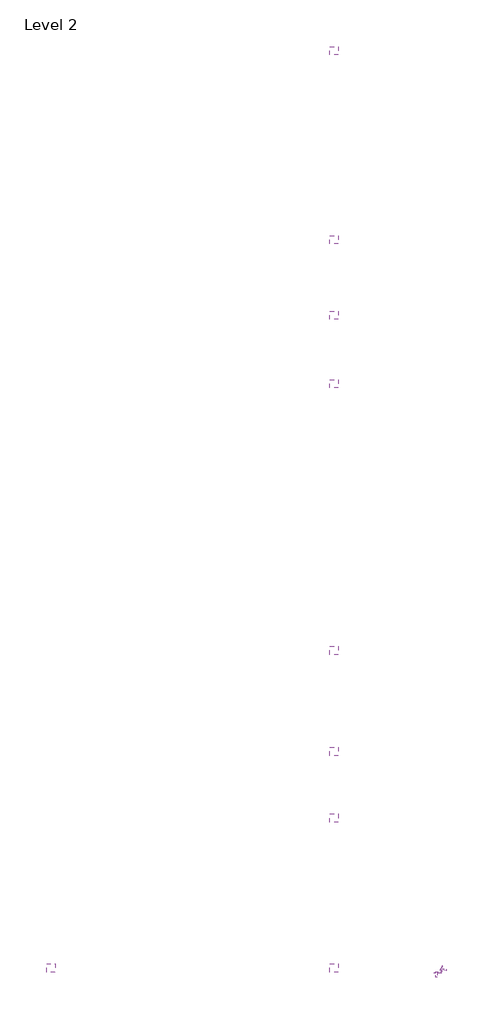
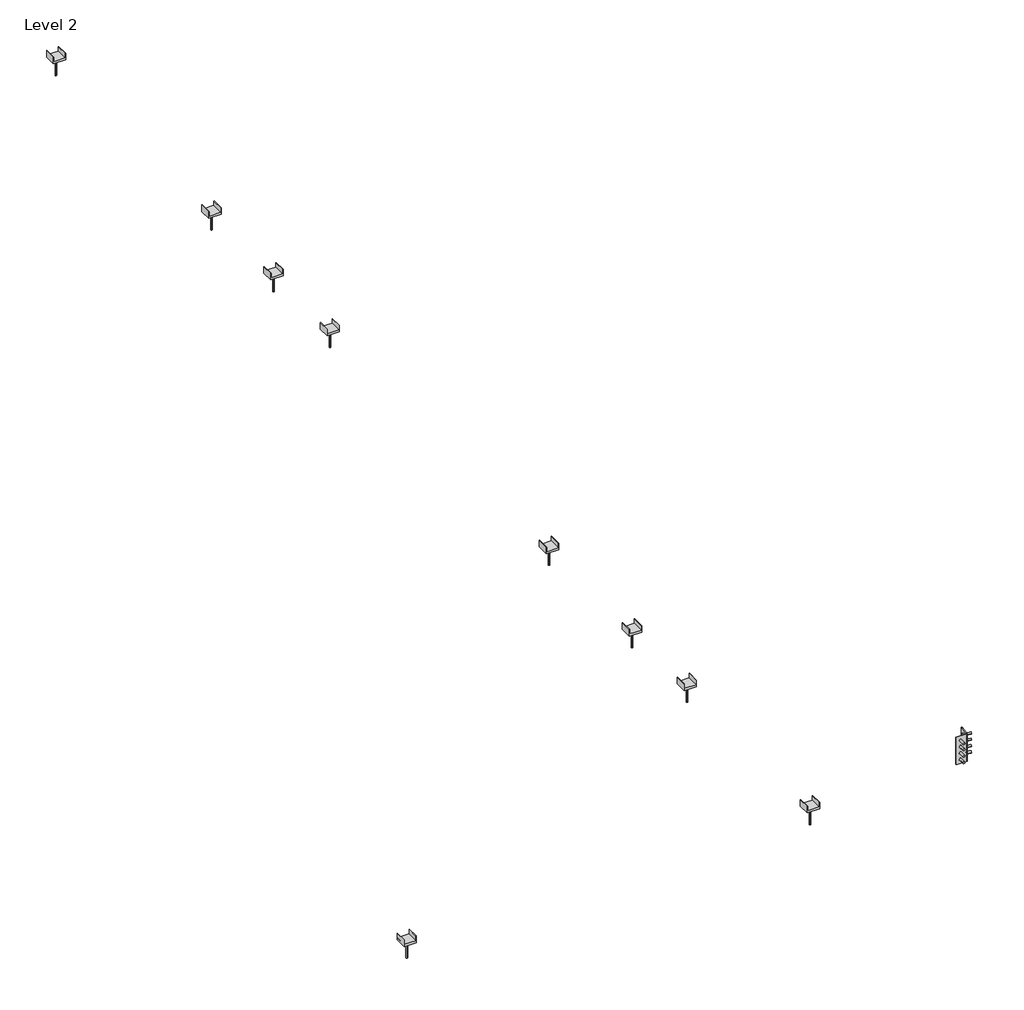
# One storey: 10 fasteners.
"""IFC4 building model written with IfcOpenShell, lengths in millimetres."""

import ifcopenshell
import ifcopenshell.guid

model = None  # the IFC model being written
_history = None  # IfcOwnerHistory: only IFC2X3 demands one
_inside = {}  # id of a spatial element -> (the spatial element, [elements in it])
_under = {}  # id of a project, library or spatial element -> (it, [spatial elements below it])
_declared = {}  # id of a project -> (the project, [libraries it declares])
_typed = {}  # id of a type object -> (the type object, [elements of that type])
_made_of = {}  # id of a material, layer set ... -> (it, [elements and type objects made of it])


def new_model(schema):
    """Start an empty IFC model of exactly this schema.

    Asked for "IFC4X3", IfcOpenShell would pick the latest addendum, in which some entities
    have other attributes; the version numbers below select the first issue.
    IFC2X3 requires an IfcOwnerHistory on every rooted entity: one is made here for all.
    """
    global model, _history
    if schema == "IFC4X3":
        model = ifcopenshell.file(schema_version=(4, 3, 0, 0))
    else:
        model = ifcopenshell.file(schema=schema)
    _inside.clear()
    _under.clear()
    _declared.clear()
    _typed.clear()
    _made_of.clear()
    _history = None
    if model.schema == "IFC2X3":
        org = make("IfcOrganization", Name="unknown")
        user = make(
            "IfcPersonAndOrganization",
            ThePerson=make("IfcPerson", FamilyName="unknown"),
            TheOrganization=org,
        )
        app = make(
            "IfcApplication",
            ApplicationDeveloper=org,
            Version="unknown",
            ApplicationFullName="unknown",
            ApplicationIdentifier="unknown",
        )
        _history = make(
            "IfcOwnerHistory",
            OwningUser=user,
            OwningApplication=app,
            ChangeAction="ADDED",
            CreationDate=0,
        )
    return model


def make(cls, **values):
    """One entity of the class cls with the attributes given. An attribute that is None is left unset."""
    return model.create_entity(
        cls, **{name: value for name, value in values.items() if value is not None}
    )


def rooted(cls, **values):
    """An entity with a GlobalId (a new one), such as an element, a storey or a relation."""
    return make(cls, GlobalId=ifcopenshell.guid.new(), OwnerHistory=_history, **values)


def si_unit(unit_type, name, prefix=None):
    """IfcSIUnit, for example si_unit("LENGTHUNIT", "METRE", prefix="MILLI")."""
    return make("IfcSIUnit", UnitType=unit_type, Prefix=prefix, Name=name)


def assignment(units):
    """IfcUnitAssignment: the units of a project."""
    return None if units is None else make("IfcUnitAssignment", Units=units)


def point(xyz):
    """IfcCartesianPoint."""
    return None if xyz is None else make("IfcCartesianPoint", Coordinates=xyz)


def direction(xyz):
    """IfcDirection."""
    return None if xyz is None else make("IfcDirection", DirectionRatios=xyz)


def frame(location, z_axis=None, x_axis=None):
    """IfcAxis2Placement3D, a coordinate frame: its origin and axes. An axis left out is left unset."""
    return make(
        "IfcAxis2Placement3D",
        Location=point(location),
        Axis=direction(z_axis),
        RefDirection=direction(x_axis),
    )


def frame_2d(location, x_axis=None):
    """IfcAxis2Placement2D, a coordinate frame in the plane: its origin and x axis."""
    return make(
        "IfcAxis2Placement2D", Location=point(location), RefDirection=direction(x_axis)
    )


def origin():
    """The frame at (0, 0, 0) with its axes left unset."""
    return frame((0.0, 0.0, 0.0))


def origin_with_axes():
    """The frame at (0, 0, 0) with the z axis (0, 0, 1) and the x axis (1, 0, 0) written out."""
    return frame((0.0, 0.0, 0.0), z_axis=(0.0, 0.0, 1.0), x_axis=(1.0, 0.0, 0.0))


def origin_2d():
    """The frame at (0, 0) in the plane with its x axis left unset."""
    return frame_2d((0.0, 0.0))


def place(relative_to, where):
    """IfcLocalPlacement: puts the frame where relative to a parent placement (None: the world)."""
    return make(
        "IfcLocalPlacement", PlacementRelTo=relative_to, RelativePlacement=where
    )


def context(
    kind, dimensions, precision=None, world=None, true_north=None, identifier=None
):
    """IfcGeometricRepresentationContext, for example the 3D "Model" context."""
    return make(
        "IfcGeometricRepresentationContext",
        ContextIdentifier=identifier,
        ContextType=kind,
        CoordinateSpaceDimension=dimensions,
        Precision=precision,
        WorldCoordinateSystem=world,
        TrueNorth=true_north,
    )


def project(units=None, contexts=None):
    """IfcProject with its units and contexts."""
    return rooted(
        "IfcProject",
        Name="project",
        RepresentationContexts=contexts,
        UnitsInContext=assignment(units),
    )


def spatial(cls, under=None, at=None, **own):
    """A site, building, storey or space (cls), placed at a placement, below another one or the project."""
    s = rooted(cls, ObjectPlacement=at, **own)
    if under is not None:
        _under.setdefault(under.id(), (under, []))[1].append(s)
    return s


def polyline(points):
    """IfcPolyline through the points."""
    return make("IfcPolyline", Points=[point(p) for p in points])


def circle_curve(where, radius):
    """IfcCircle in the frame where."""
    return make("IfcCircle", Position=where, Radius=radius)


def trimmed(basis, trim1, trim2, sense, master):
    """IfcTrimmedCurve: the piece of a basis curve between two trims."""
    return make(
        "IfcTrimmedCurve",
        BasisCurve=basis,
        Trim1=trim1,
        Trim2=trim2,
        SenseAgreement=sense,
        MasterRepresentation=master,
    )


def segment(curve, same_sense, transition):
    """IfcCompositeCurveSegment."""
    return make(
        "IfcCompositeCurveSegment",
        Transition=transition,
        SameSense=same_sense,
        ParentCurve=curve,
    )


def composite_curve(segments, self_intersect=None):
    """IfcCompositeCurve: segments joined end to end."""
    return make("IfcCompositeCurve", Segments=segments, SelfIntersect=self_intersect)


def outline(outer, holes=None, kind="AREA"):
    """IfcArbitraryClosedProfileDef: a profile drawn as a closed curve; with holes, ...WithVoids."""
    if holes is None:
        return make("IfcArbitraryClosedProfileDef", ProfileType=kind, OuterCurve=outer)
    return make(
        "IfcArbitraryProfileDefWithVoids",
        ProfileType=kind,
        OuterCurve=outer,
        InnerCurves=holes,
    )


def extrude(swept, where, along, depth):
    """IfcExtrudedAreaSolid: the profile swept, set in the frame where, extruded along a direction by depth."""
    return make(
        "IfcExtrudedAreaSolid",
        SweptArea=swept,
        Position=where,
        ExtrudedDirection=direction(along),
        Depth=depth,
    )


def shape(context_of_items, identifier, shape_type, items):
    """IfcShapeRepresentation: the items that make up one representation, for example the "Body"."""
    return make(
        "IfcShapeRepresentation",
        ContextOfItems=context_of_items,
        RepresentationIdentifier=identifier,
        RepresentationType=shape_type,
        Items=items,
    )


def source(mapping_origin, context_of_items, identifier, shape_type, items):
    """IfcRepresentationMap: a shape defined once, which mapped items show again and again."""
    return make(
        "IfcRepresentationMap",
        MappingOrigin=mapping_origin,
        MappedRepresentation=shape(context_of_items, identifier, shape_type, items),
    )


def transform(
    local_origin,
    x_axis=None,
    y_axis=None,
    z_axis=None,
    scale=None,
    scale2=None,
    scale3=None,
    uniform=True,
):
    """IfcCartesianTransformationOperator3D, or its non-uniform kind. x_axis, y_axis, z_axis: its Axis1, 2, 3."""
    if uniform:
        return make(
            "IfcCartesianTransformationOperator3D",
            Axis1=direction(x_axis),
            Axis2=direction(y_axis),
            LocalOrigin=point(local_origin),
            Scale=scale,
            Axis3=direction(z_axis),
        )
    return make(
        "IfcCartesianTransformationOperator3DnonUniform",
        Axis1=direction(x_axis),
        Axis2=direction(y_axis),
        LocalOrigin=point(local_origin),
        Scale=scale,
        Axis3=direction(z_axis),
        Scale2=scale2,
        Scale3=scale3,
    )


def mapped(mapping_source, mapping_target):
    """IfcMappedItem: shows the shape of a source again, moved by a transform."""
    return make(
        "IfcMappedItem", MappingSource=mapping_source, MappingTarget=mapping_target
    )


def made_of(thing, what):
    """Note that an element or type object is made of a material, layer set ...; save() writes the relation."""
    if what is not None:
        _made_of.setdefault(what.id(), (what, []))[1].append(thing)
    return thing


def element(
    cls,
    number,
    at=None,
    inside=None,
    cuts=None,
    type_object=None,
    material=None,
    context=None,
    identifier="Body",
    shape_type=None,
    held_by="IfcProductDefinitionShape",
    body=None,
    shapes=None,
    **own,
):
    """One element of the class cls, such as IfcWall. Its Tag is "e" and its number.

    at: its placement. inside: the storey or other place that contains it. cuts: it is an
    opening in that element (IfcRelVoidsElement). A single representation is given by context,
    identifier, shape_type and body (its items); several are given by shapes. held_by: the class
    of the entity that holds the representations. save() writes the other relations.
    """
    e = rooted(cls, Tag="e%d" % number, ObjectPlacement=at, **own)
    if body is not None:
        shapes = [shape(context, identifier, shape_type, body)]
    if shapes is not None:
        e.Representation = make(held_by, Representations=shapes)
    if inside is not None:
        _inside.setdefault(inside.id(), (inside, []))[1].append(e)
    if cuts is not None:
        rooted(
            "IfcRelVoidsElement", RelatingBuildingElement=cuts, RelatedOpeningElement=e
        )
    if type_object is not None:
        _typed.setdefault(type_object.id(), (type_object, []))[1].append(e)
    return made_of(e, material)


def aggregate(whole, parts):
    """IfcRelAggregates: a whole, such as a stair, and the parts it consists of."""
    return rooted("IfcRelAggregates", RelatingObject=whole, RelatedObjects=parts)


def save(model, path):
    """Write the relations noted so far, then the file.

    IfcRelAggregates (storeys below a building ...), IfcRelContainedInSpatialStructure (elements
    in a storey), IfcRelDefinesByType, IfcRelAssociatesMaterial and IfcRelDeclares: one each for
    every whole, place, type object, material and project.
    """
    for whole, parts in _under.values():
        aggregate(whole, parts)
    for where, things in _inside.values():
        rooted(
            "IfcRelContainedInSpatialStructure",
            RelatedElements=things,
            RelatingStructure=where,
        )
    for kind, things in _typed.values():
        rooted("IfcRelDefinesByType", RelatedObjects=things, RelatingType=kind)
    for what, things in _made_of.values():
        rooted("IfcRelAssociatesMaterial", RelatedObjects=things, RelatingMaterial=what)
    for by, libraries in _declared.values():
        rooted("IfcRelDeclares", RelatingContext=by, RelatedDefinitions=libraries)
    model.write(path)


def plane_surface(at):
    """IfcPlane: the flat surface through the origin of the frame at, square to its z axis."""
    return make("IfcPlane", Position=at)


def revolved_surface(curve, axis_point, axis_direction):
    """IfcSurfaceOfRevolution: the curve turned about the line through axis_point along axis_direction."""
    return make(
        "IfcSurfaceOfRevolution",
        SweptCurve=make("IfcArbitraryOpenProfileDef", ProfileType="CURVE", Curve=curve),
        AxisPosition=make("IfcAxis1Placement", Location=point(axis_point), Axis=direction(axis_direction)),
    )


def advanced_brep(points, edges, surfaces, faces):
    """IfcAdvancedBrep: a solid bounded by faces that lie on surfaces and meet in shared edges.

    An edge is (start, end): straight between two places in points (the first is 0);
    or (start, end, curve); or (start, end, curve, False) where it runs against its curve.
    A face is (place in surfaces, loops), or (place, loops, False) where it looks against
    its surface's normal. A loop lists edges by number (the first is 1), with a minus sign
    where the edge is run from its end to its start. The first loop is the outer one.
    """
    corners = [point(p) for p in points]
    vertices = [make("IfcVertexPoint", VertexGeometry=c) for c in corners]
    made = []
    for start, end, *more in edges:
        made.append(
            make(
                "IfcEdgeCurve",
                EdgeStart=vertices[start],
                EdgeEnd=vertices[end],
                EdgeGeometry=more[0] if more else make("IfcPolyline", Points=[corners[start], corners[end]]),
                SameSense=more[1] if len(more) > 1 else True,
            )
        )
    hull = []
    for where, loops, *sense in faces:
        bounds = []
        for j, loop in enumerate(loops):
            ring = [make("IfcOrientedEdge", EdgeElement=made[abs(k) - 1], Orientation=k > 0) for k in loop]
            bounds.append(
                make(
                    "IfcFaceOuterBound" if j == 0 else "IfcFaceBound",
                    Bound=make("IfcEdgeLoop", EdgeList=ring),
                    Orientation=True,
                )
            )
        hull.append(make("IfcAdvancedFace", Bounds=bounds, FaceSurface=surfaces[where], SameSense=sense[0] if sense else True))
    return make("IfcAdvancedBrep", Outer=make("IfcClosedShell", CfsFaces=hull))


def fastener_d5b4f6b8(model_context):
    return source(origin(), model_context, "Body", "SweptSolid", [
        extrude(outline(composite_curve([segment(trimmed(circle_curve(origin_2d(), 7.9375), [point((-7.9375, 0.0))], [point((7.9375, 0.0))], False, "CARTESIAN"), True, "CONTINUOUS"), segment(trimmed(circle_curve(origin_2d(), 7.9375), [point((7.9375, 0.0))], [point((-7.9375, 0.0))], False, "CARTESIAN"), True, "CONTINUOUS")], self_intersect=False)), frame((0.0, 0.0, -203.2), z_axis=(0.0, 0.0, 1.0), x_axis=(1.0, 0.0, 0.0)), (0.0, 0.0, 1.0), 203.2),
        extrude(outline(polyline([(-11.90625, 6.8740766), (0.0, 13.7481533), (11.90625, 6.8740766), (11.90625, -6.8740766), (0.0, -13.7481533), (-11.90625, -6.8740766), (-11.90625, 6.8740766)])), origin_with_axes(), (0.0, 0.0, 1.0), 11.2117187),
        extrude(outline(polyline([(-69.85, 79.375), (-66.675, 79.375), (-66.675, 25.4), (66.675, 25.4), (66.675, 79.375), (69.85, 79.375), (69.85, 0.0), (-69.85, 0.0), (-69.85, 79.375)])), frame((-68.2625, 0.0, 0.0), z_axis=(1.0, 0.0, 0.0), x_axis=(0.0, 1.0, 0.0)), (0.0, 0.0, 1.0), 136.525),
    ])


def fastener_ec502d19(model_context):
    return source(origin(), model_context, "Body", "SweptSolid", [
        extrude(outline(composite_curve([segment(trimmed(circle_curve(origin_2d(), 7.9375), [point((-7.9375, 0.0))], [point((7.9375, 0.0))], False, "CARTESIAN"), True, "CONTINUOUS"), segment(trimmed(circle_curve(origin_2d(), 7.9375), [point((7.9375, 0.0))], [point((-7.9375, 0.0))], False, "CARTESIAN"), True, "CONTINUOUS")], self_intersect=False)), frame((0.0, 0.0, -203.2), z_axis=(0.0, 0.0, 1.0), x_axis=(1.0, 0.0, 0.0)), (0.0, 0.0, 1.0), 203.2),
        extrude(outline(polyline([(-11.90625, -6.8740766), (-11.90625, 6.8740766), (0.0, 13.7481533), (11.90625, 6.8740766), (11.90625, -6.8740766), (0.0, -13.7481533), (-11.90625, -6.8740766)])), origin_with_axes(), (0.0, 0.0, 1.0), 11.2117187),
        extrude(outline(polyline([(69.85, 79.375), (69.85, 0.0), (-69.85, 0.0), (-69.85, 79.375), (-66.675, 79.375), (-66.675, 25.4), (66.675, 25.4), (66.675, 79.375), (69.85, 79.375)])), frame((-68.2625, 0.0, 0.0), z_axis=(1.0, 0.0, 0.0), x_axis=(0.0, 1.0, 0.0)), (0.0, 0.0, 1.0), 136.525),
    ])


def corner_bracket_angled_dba65dea(model_context):
    return source(origin(), model_context, "Body", "SolidModel", [
        advanced_brep(
        [(65.484375, -7.9375, 203.2), (65.484375, 0.0, 203.2), (93.265625, 0.0, 203.2), (93.265625, -7.9375, 203.2), (93.265625, -7.9375, 279.4), (93.265625, 0.0, 279.4), (65.484375, 0.0, 279.4), (65.484375, -7.9375, 279.4), (127.0, 0.0, 0.0), (127.0, 0.0, 330.2), (127.0, -7.9375, 330.2), (127.0, -7.9375, 0.0), (65.484375, -7.9375, 127.0), (65.484375, 0.0, 127.0), (93.265625, 0.0, 127.0), (93.265625, -7.9375, 127.0), (65.484375, -7.9375, 50.8), (65.484375, 0.0, 50.8), (93.265625, 0.0, 50.8), (93.265625, -7.9375, 50.8), (7.1469571, -7.9375, 330.2), (7.1469571, -7.9375, 0.0), (0.0, 0.0, 0.0), (0.0, 0.0, 330.2), (7.8940175, -0.8296947, 330.2), (7.8940175, -0.8296947, 0.0)],
        [
            (0, 1),
            (1, 2, circle_curve(frame((79.375, 0.0, 203.2), z_axis=(0.0, 1.0, 0.0), x_axis=(-1.0000000000000002, 0.0, 0.0)), 13.890625)),
            (2, 3),
            (3, 0, circle_curve(frame((79.375, -7.9375, 203.2), z_axis=(0.0, -1.0, 0.0), x_axis=(-1.0000000000000002, 0.0, 0.0)), 13.890625)),
            (4, 5),
            (5, 6, circle_curve(frame((79.375, 0.0, 279.4), z_axis=(0.0, 1.0, 0.0), x_axis=(-1.0000000000000002, 0.0, 0.0)), 13.890625)),
            (6, 7),
            (7, 4, circle_curve(frame((79.375, -7.9375, 279.4), z_axis=(0.0, -1.0, 0.0), x_axis=(-1.0000000000000002, 0.0, 0.0)), 13.890625)),
            (8, 9),
            (9, 10),
            (10, 11),
            (11, 8),
            (6, 5, circle_curve(frame((79.375, 0.0, 279.4), z_axis=(0.0, 1.0, 0.0), x_axis=(-1.0000000000000002, 0.0, 0.0)), 13.890625)),
            (4, 7, circle_curve(frame((79.375, -7.9375, 279.4), z_axis=(0.0, -1.0, 0.0), x_axis=(-1.0000000000000002, 0.0, 0.0)), 13.890625)),
            (12, 13),
            (13, 14, circle_curve(frame((79.375, 0.0, 127.0), z_axis=(0.0, 1.0, 0.0), x_axis=(-1.0000000000000002, 0.0, 0.0)), 13.890625)),
            (14, 15),
            (15, 12, circle_curve(frame((79.375, -7.9375, 127.0), z_axis=(0.0, -1.0, 0.0), x_axis=(-1.0000000000000002, 0.0, 0.0)), 13.890625)),
            (16, 17),
            (17, 18, circle_curve(frame((79.375, 0.0, 50.8), z_axis=(0.0, 1.0, 0.0), x_axis=(-1.0000000000000002, 0.0, 0.0)), 13.890625)),
            (18, 19),
            (19, 16, circle_curve(frame((79.375, -7.9375, 50.8), z_axis=(0.0, -1.0, 0.0), x_axis=(-1.0000000000000002, 0.0, 0.0)), 13.890625)),
            (10, 20),
            (20, 21),
            (21, 11),
            (3, 0, circle_curve(frame((79.375, -7.9375, 203.2), z_axis=(0.0, 1.0, 0.0), x_axis=(-1.0000000000000002, 0.0, 0.0)), 13.890625)),
            (15, 12, circle_curve(frame((79.375, -7.9375, 127.0), z_axis=(0.0, 1.0, 0.0), x_axis=(-1.0000000000000002, 0.0, 0.0)), 13.890625)),
            (19, 16, circle_curve(frame((79.375, -7.9375, 50.8), z_axis=(0.0, 1.0, 0.0), x_axis=(-1.0000000000000002, 0.0, 0.0)), 13.890625)),
            (8, 22),
            (22, 23),
            (23, 9),
            (1, 2, circle_curve(frame((79.375, 0.0, 203.2), z_axis=(0.0, -1.0, 0.0), x_axis=(-1.0000000000000002, 0.0, 0.0)), 13.890625)),
            (13, 14, circle_curve(frame((79.375, 0.0, 127.0), z_axis=(0.0, -1.0, 0.0), x_axis=(-1.0000000000000002, 0.0, 0.0)), 13.890625)),
            (17, 18, circle_curve(frame((79.375, 0.0, 50.8), z_axis=(0.0, -1.0, 0.0), x_axis=(-1.0000000000000002, 0.0, 0.0)), 13.890625)),
            (23, 24),
            (24, 20),
            (21, 25),
            (25, 22),
            (24, 25),
        ],
        [
            revolved_surface(polyline([(65.484375, -7.937500000000007, 203.2), (65.484375, 0.0, 203.2)]), (79.375, 0.0, 203.2), (0.0, -1.0000000000000004, 0.0)),
            revolved_surface(polyline([(65.484375, -7.937500000000007, 279.4), (65.484375, 0.0, 279.4)]), (79.375, 0.0, 279.4), (0.0, -1.0000000000000004, 0.0)),
            plane_surface(frame((127.0, -7.9375, 330.2), z_axis=(1.0, 0.0, 0.0), x_axis=(0.0, 1.0, 0.0))),
            revolved_surface(polyline([(65.484375, -7.937500000000007, 127.0), (65.484375, 0.0, 127.0)]), (79.375, 0.0, 127.0), (0.0, -1.0000000000000004, 0.0)),
            revolved_surface(polyline([(65.484375, -7.937500000000007, 50.8), (65.484375, 0.0, 50.8)]), (79.375, 0.0, 50.8), (0.0, -1.0000000000000004, 0.0)),
            plane_surface(frame((127.0, -7.9375, 330.2), z_axis=(0.0, -1.0, 0.0), x_axis=(1.0, 0.0, 0.0))),
            plane_surface(frame((127.0, 0.0, 330.2), z_axis=(0.0, 1.0, 0.0), x_axis=(-1.0, 0.0, 0.0))),
            plane_surface(frame((0.0, -7.9375, 330.2), z_axis=(0.0, 0.0, 1.0), x_axis=(0.0, 1.0, 0.0))),
            plane_surface(frame((127.0, -7.9375, 0.0), z_axis=(0.0, 0.0, -1.0), x_axis=(0.0, 1.0, 0.0))),
            plane_surface(frame((-5.3810973, -127.1339754, 330.2), z_axis=(-0.9945218953682736, 0.10452846326765133, 0.0), x_axis=(-0.10452846326765133, -0.9945218953682736, 0.0))),
            plane_surface(frame((7.8940175, -0.8296947, 0.0), z_axis=(-0.10452846326765133, -0.9945218953682736, 0.0), x_axis=(-0.9945218953682736, 0.10452846326765133, 0.0))),
        ],
        [
            (0, [[1, 2, 3, 4]]),
            (1, [[5, 6, 7, 8]]),
            (2, [[9, 10, 11, 12]]),
            (1, [[-7, 13, -5, 14]]),
            (3, [[15, 16, 17, 18]]),
            (4, [[19, 20, 21, 22]]),
            (5, [[23, 24, 25, -11], [-14, -8], [-4, 26], [-18, 27], [-22, 28]]),
            (6, [[-9, 29, 30, 31], [-2, 32], [-16, 33], [-13, -6], [-20, 34]]),
            (7, [[35, 36, -23, -10, -31]]),
            (8, [[-25, 37, 38, -29, -12]]),
            (0, [[-3, -32, -1, -26]]),
            (3, [[-17, -33, -15, -27]]),
            (4, [[-21, -34, -19, -28]]),
            (9, [[-37, -24, -36, 39]]),
            (10, [[-35, -30, -38, -39]]),
        ],
    ),
        extrude(outline(polyline([(290.3985226, 98.425), (301.3970453, 79.375), (290.3985226, 60.325), (268.4014774, 60.325), (257.4029547, 79.375), (268.4014774, 98.425), (290.3985226, 98.425)])), frame((0.0, -22.9195312, 0.0), z_axis=(0.0, 1.0, 0.0), x_axis=(0.0, 0.0, 1.0)), (0.0, 0.0, 1.0), 14.9820312),
        extrude(outline(composite_curve([segment(trimmed(circle_curve(frame_2d((279.4, 79.375)), 12.7), [point((279.4, 92.075))], [point((279.4, 66.675))], False, "CARTESIAN"), True, "CONTINUOUS"), segment(trimmed(circle_curve(frame_2d((279.4, 79.375)), 12.7), [point((279.4, 66.675))], [point((279.4, 92.075))], False, "CARTESIAN"), True, "CONTINUOUS")], self_intersect=False)), frame((0.0, -7.9375, 0.0), z_axis=(0.0, 1.0, 0.0), x_axis=(0.0, 0.0, 1.0)), (0.0, 0.0, 1.0), 76.2),
        extrude(outline(polyline([(214.1985226, 98.425), (225.1970453, 79.375), (214.1985226, 60.325), (192.2014774, 60.325), (181.2029547, 79.375), (192.2014774, 98.425), (214.1985226, 98.425)])), frame((0.0, -22.9195312, 0.0), z_axis=(0.0, 1.0, 0.0), x_axis=(0.0, 0.0, 1.0)), (0.0, 0.0, 1.0), 14.9820312),
        extrude(outline(composite_curve([segment(trimmed(circle_curve(frame_2d((203.2, 79.375)), 12.7), [point((203.2, 92.075))], [point((203.2, 66.675))], False, "CARTESIAN"), True, "CONTINUOUS"), segment(trimmed(circle_curve(frame_2d((203.2, 79.375)), 12.7), [point((203.2, 66.675))], [point((203.2, 92.075))], False, "CARTESIAN"), True, "CONTINUOUS")], self_intersect=False)), frame((0.0, -7.9375, 0.0), z_axis=(0.0, 1.0, 0.0), x_axis=(0.0, 0.0, 1.0)), (0.0, 0.0, 1.0), 76.2),
        extrude(outline(polyline([(290.3985226, 98.425), (301.3970453, 79.375), (290.3985226, 60.325), (268.4014774, 60.325), (257.4029547, 79.375), (268.4014774, 98.425), (290.3985226, 98.425)])), frame((0.0, -22.9195312, 0.0), z_axis=(0.0, 1.0, 0.0), x_axis=(0.0, 0.0, 1.0)), (0.0, 0.0, 1.0), 14.9820312),
        extrude(outline(composite_curve([segment(trimmed(circle_curve(frame_2d((279.4, 79.375)), 12.7), [point((279.4, 92.075))], [point((279.4, 66.675))], False, "CARTESIAN"), True, "CONTINUOUS"), segment(trimmed(circle_curve(frame_2d((279.4, 79.375)), 12.7), [point((279.4, 66.675))], [point((279.4, 92.075))], False, "CARTESIAN"), True, "CONTINUOUS")], self_intersect=False)), frame((0.0, -7.9375, 0.0), z_axis=(0.0, 1.0, 0.0), x_axis=(0.0, 0.0, 1.0)), (0.0, 0.0, 1.0), 76.2),
        extrude(outline(polyline([(137.9985226, 98.425), (148.9970453, 79.375), (137.9985226, 60.325), (116.0014774, 60.325), (105.0029547, 79.375), (116.0014774, 98.425), (137.9985226, 98.425)])), frame((0.0, -22.9195312, 0.0), z_axis=(0.0, 1.0, 0.0), x_axis=(0.0, 0.0, 1.0)), (0.0, 0.0, 1.0), 14.9820312),
        extrude(outline(composite_curve([segment(trimmed(circle_curve(frame_2d((127.0, 79.375)), 12.7), [point((127.0, 92.075))], [point((127.0, 66.675))], False, "CARTESIAN"), True, "CONTINUOUS"), segment(trimmed(circle_curve(frame_2d((127.0, 79.375)), 12.7), [point((127.0, 66.675))], [point((127.0, 92.075))], False, "CARTESIAN"), True, "CONTINUOUS")], self_intersect=False)), frame((0.0, -7.9375, 0.0), z_axis=(0.0, 1.0, 0.0), x_axis=(0.0, 0.0, 1.0)), (0.0, 0.0, 1.0), 76.2),
        extrude(outline(polyline([(61.7985226, 98.425), (72.7970453, 79.375), (61.7985226, 60.325), (39.8014774, 60.325), (28.8029547, 79.375), (39.8014774, 98.425), (61.7985226, 98.425)])), frame((0.0, -22.9195312, 0.0), z_axis=(0.0, 1.0, 0.0), x_axis=(0.0, 0.0, 1.0)), (0.0, 0.0, 1.0), 14.9820312),
        extrude(outline(composite_curve([segment(trimmed(circle_curve(frame_2d((50.8, 79.375)), 12.7), [point((50.8, 92.075))], [point((50.8, 66.675))], False, "CARTESIAN"), True, "CONTINUOUS"), segment(trimmed(circle_curve(frame_2d((50.8, 79.375)), 12.7), [point((50.8, 66.675))], [point((50.8, 92.075))], False, "CARTESIAN"), True, "CONTINUOUS")], self_intersect=False)), frame((0.0, -7.9375, 0.0), z_axis=(0.0, 1.0, 0.0), x_axis=(0.0, 0.0, 1.0)), (0.0, 0.0, 1.0), 76.2),
        advanced_brep(
        [(-0.1955056, -77.7963657, 203.2), (-8.0895231, -76.9666711, 203.2), (-5.1855917, -49.3376097, 203.2), (2.7084258, -50.1673043, 203.2), (-8.0895231, -76.9666711, 279.4), (-0.1955056, -77.7963657, 279.4), (2.7084258, -50.1673043, 279.4), (-5.1855917, -49.3376097, 279.4), (-5.3810973, -127.1339754, 0.0), (-5.3810973, -127.1339754, 330.2), (-13.2751148, -126.3042807, 330.2), (-13.2751148, -126.3042807, 0.0), (-0.1955056, -77.7963657, 127.0), (-8.0895231, -76.9666711, 127.0), (-5.1855917, -49.3376097, 127.0), (2.7084258, -50.1673043, 127.0), (-0.1955056, -77.7963657, 50.8), (-8.0895231, -76.9666711, 50.8), (-5.1855917, -49.3376097, 50.8), (2.7084258, -50.1673043, 50.8), (7.8940175, -0.8296947, 330.2), (7.1469571, -7.9375, 330.2), (7.1469571, -7.9375, 0.0), (7.8940175, -0.8296947, 0.0), (0.0, 0.0, 330.2), (0.0, 0.0, 0.0)],
        [
            (0, 1),
            (1, 2, circle_curve(frame((-6.6375574, -63.1521404, 203.2), z_axis=(-0.9945218953682737, 0.10452846326765135, 0.0), x_axis=(0.10452846326765132, 0.9945218953682735, 0.0)), 13.890625)),
            (2, 3),
            (3, 0, circle_curve(frame((1.2564601, -63.981835, 203.2), z_axis=(0.9945218953682737, -0.10452846326765135, 0.0), x_axis=(0.10452846326765132, 0.9945218953682735, 0.0)), 13.890625)),
            (4, 5),
            (5, 6, circle_curve(frame((1.2564601, -63.981835, 279.4), z_axis=(0.9945218953682737, -0.10452846326765135, 0.0), x_axis=(0.10452846326765132, 0.9945218953682735, 0.0)), 13.890625)),
            (6, 7),
            (7, 4, circle_curve(frame((-6.6375574, -63.1521404, 279.4), z_axis=(-0.9945218953682737, 0.10452846326765135, 0.0), x_axis=(0.10452846326765132, 0.9945218953682735, 0.0)), 13.890625)),
            (8, 9),
            (9, 10),
            (10, 11),
            (11, 8),
            (4, 7, circle_curve(frame((-6.6375574, -63.1521404, 279.4), z_axis=(-0.9945218953682737, 0.10452846326765135, 0.0), x_axis=(0.10452846326765132, 0.9945218953682735, 0.0)), 13.890625)),
            (6, 5, circle_curve(frame((1.2564601, -63.981835, 279.4), z_axis=(0.9945218953682737, -0.10452846326765135, 0.0), x_axis=(0.10452846326765132, 0.9945218953682735, 0.0)), 13.890625)),
            (12, 13),
            (13, 14, circle_curve(frame((-6.6375574, -63.1521404, 127.0), z_axis=(-0.9945218953682737, 0.10452846326765135, 0.0), x_axis=(0.10452846326765132, 0.9945218953682735, 0.0)), 13.890625)),
            (14, 15),
            (15, 12, circle_curve(frame((1.2564601, -63.981835, 127.0), z_axis=(0.9945218953682737, -0.10452846326765135, 0.0), x_axis=(0.10452846326765132, 0.9945218953682735, 0.0)), 13.890625)),
            (16, 17),
            (17, 18, circle_curve(frame((-6.6375574, -63.1521404, 50.8), z_axis=(-0.9945218953682737, 0.10452846326765135, 0.0), x_axis=(0.10452846326765132, 0.9945218953682735, 0.0)), 13.890625)),
            (18, 19),
            (19, 16, circle_curve(frame((1.2564601, -63.981835, 50.8), z_axis=(0.9945218953682737, -0.10452846326765135, 0.0), x_axis=(0.10452846326765132, 0.9945218953682735, 0.0)), 13.890625)),
            (20, 21),
            (21, 9),
            (8, 22),
            (22, 23),
            (23, 20),
            (19, 16, circle_curve(frame((1.2564601, -63.981835, 50.8), z_axis=(-0.9945218953682737, 0.10452846326765135, 0.0), x_axis=(0.10452846326765132, 0.9945218953682735, 0.0)), 13.890625)),
            (15, 12, circle_curve(frame((1.2564601, -63.981835, 127.0), z_axis=(-0.9945218953682737, 0.10452846326765135, 0.0), x_axis=(0.10452846326765132, 0.9945218953682735, 0.0)), 13.890625)),
            (3, 0, circle_curve(frame((1.2564601, -63.981835, 203.2), z_axis=(-0.9945218953682737, 0.10452846326765135, 0.0), x_axis=(0.10452846326765132, 0.9945218953682735, 0.0)), 13.890625)),
            (24, 25),
            (25, 11),
            (10, 24),
            (1, 2, circle_curve(frame((-6.6375574, -63.1521404, 203.2), z_axis=(0.9945218953682737, -0.10452846326765135, 0.0), x_axis=(0.10452846326765132, 0.9945218953682735, 0.0)), 13.890625)),
            (17, 18, circle_curve(frame((-6.6375574, -63.1521404, 50.8), z_axis=(0.9945218953682737, -0.10452846326765135, 0.0), x_axis=(0.10452846326765132, 0.9945218953682735, 0.0)), 13.890625)),
            (13, 14, circle_curve(frame((-6.6375574, -63.1521404, 127.0), z_axis=(0.9945218953682737, -0.10452846326765135, 0.0), x_axis=(0.10452846326765132, 0.9945218953682735, 0.0)), 13.890625)),
            (20, 24),
            (25, 23),
        ],
        [
            revolved_surface(polyline([(2.7084257925952384, -50.1673043704516, 203.2), (-5.1855917299787775, -49.33760969556763, 203.2)]), (-6.6375574, -63.1521404, 203.2), (0.9945218953682735, -0.10452846326765132, 0.0)),
            revolved_surface(polyline([(2.7084257925952384, -50.1673043704516, 279.4), (-5.1855917299787775, -49.33760969556763, 279.4)]), (-6.6375574, -63.1521404, 279.4), (0.9945218953682735, -0.10452846326765132, 0.0)),
            plane_surface(frame((-5.3810973, -127.1339754, 330.2), z_axis=(-0.10452846326765133, -0.9945218953682736, 0.0), x_axis=(-0.9945218953682736, 0.10452846326765133, 0.0))),
            revolved_surface(polyline([(2.7084257925952384, -50.1673043704516, 127.0), (-5.1855917299787775, -49.33760969556763, 127.0)]), (-6.6375574, -63.1521404, 127.0), (0.9945218953682735, -0.10452846326765132, 0.0)),
            revolved_surface(polyline([(2.7084257925952384, -50.1673043704516, 50.8), (-5.1855917299787775, -49.33760969556763, 50.8)]), (-6.6375574, -63.1521404, 50.8), (0.9945218953682735, -0.10452846326765132, 0.0)),
            plane_surface(frame((-5.3810973, -127.1339754, 330.2), z_axis=(0.9945218953682736, -0.10452846326765133, 0.0), x_axis=(-0.10452846326765133, -0.9945218953682736, 0.0))),
            plane_surface(frame((-13.2751148, -126.3042807, 330.2), z_axis=(-0.9945218953682736, 0.10452846326765133, 0.0), x_axis=(0.10452846326765133, 0.9945218953682736, 0.0))),
            plane_surface(frame((7.8940175, -0.8296947, 330.2), z_axis=(0.0, 0.0, 1.0000000000000002), x_axis=(-0.9945218953682736, 0.10452846326765133, 0.0))),
            plane_surface(frame((-5.3810973, -127.1339754, 0.0), z_axis=(0.0, 0.0, -1.0000000000000002), x_axis=(-0.9945218953682736, 0.10452846326765133, 0.0))),
            plane_surface(frame((7.8940175, -0.8296947, 0.0), z_axis=(0.10452846326765133, 0.9945218953682736, 0.0), x_axis=(-0.9945218953682736, 0.10452846326765133, 0.0))),
        ],
        [
            (0, [[1, 2, 3, 4]]),
            (1, [[5, 6, 7, 8]]),
            (2, [[9, 10, 11, 12]]),
            (1, [[-5, 13, -7, 14]]),
            (3, [[15, 16, 17, 18]]),
            (4, [[19, 20, 21, 22]]),
            (5, [[23, 24, -9, 25, 26, 27], [-6, -14], [28, -22], [29, -18], [30, -4]]),
            (6, [[31, 32, -11, 33], [34, -2], [35, -20], [-8, -13], [36, -16]]),
            (7, [[-24, -23, 37, -33, -10]]),
            (8, [[-26, -25, -12, -32, 38]]),
            (9, [[-27, -38, -31, -37]]),
            (0, [[-1, -30, -3, -34]]),
            (3, [[-15, -29, -17, -36]]),
            (4, [[-19, -28, -21, -35]]),
        ],
    ),
        extrude(outline(polyline([(0.0, 0.0), (21.9970452, 0.0), (32.9955679, -19.05), (21.9970452, -38.1), (0.0, -38.1), (-10.9985227, -19.05), (0.0, 0.0)])), frame((14.165151, -84.4935258, 290.3985226), z_axis=(-0.9945218953682736, 0.10452846326765133, 0.0), x_axis=(0.0, 0.0, -1.0)), (0.0, 0.0, 1.0), 14.9820312),
        extrude(outline(composite_curve([segment(trimmed(circle_curve(frame_2d((0.0, -12.6999999)), 12.7), [point((0.0, -25.4))], [point((0.0, 0.0))], False, "CARTESIAN"), True, "CONTINUOUS"), segment(trimmed(circle_curve(frame_2d((0.0, -12.6999999)), 12.7), [point((0.0, 0.0))], [point((0.0, -25.4))], False, "CARTESIAN"), True, "CONTINUOUS")], self_intersect=False)), frame((2.5839716, -51.351407, 279.4), z_axis=(-0.9945218953682736, 0.10452846326765133, 0.0), x_axis=(0.0, 0.0, 1.0)), (0.0, 0.0, 1.0), 76.2),
        extrude(outline(polyline([(0.0, 0.0), (21.9970452, 0.0), (32.9955679, -19.05), (21.9970452, -38.1), (0.0, -38.1), (-10.9985227, -19.05), (0.0, 0.0)])), frame((14.165151, -84.4935258, 214.1985226), z_axis=(-0.9945218953682736, 0.10452846326765133, 0.0), x_axis=(0.0, 0.0, -1.0)), (0.0, 0.0, 1.0), 14.9820312),
        extrude(outline(composite_curve([segment(trimmed(circle_curve(frame_2d((0.0, -12.6999999)), 12.7), [point((0.0, -25.4))], [point((0.0, 0.0))], False, "CARTESIAN"), True, "CONTINUOUS"), segment(trimmed(circle_curve(frame_2d((0.0, -12.6999999)), 12.7), [point((0.0, 0.0))], [point((0.0, -25.4))], False, "CARTESIAN"), True, "CONTINUOUS")], self_intersect=False)), frame((2.5839716, -51.351407, 203.2), z_axis=(-0.9945218953682736, 0.10452846326765133, 0.0), x_axis=(0.0, 0.0, 1.0)), (0.0, 0.0, 1.0), 76.2),
        extrude(outline(polyline([(0.0, 0.0), (21.9970452, 0.0), (32.9955679, -19.05), (21.9970452, -38.1), (0.0, -38.1), (-10.9985227, -19.05), (0.0, 0.0)])), frame((14.165151, -84.4935258, 290.3985226), z_axis=(-0.9945218953682736, 0.10452846326765133, 0.0), x_axis=(0.0, 0.0, -1.0)), (0.0, 0.0, 1.0), 14.9820312),
        extrude(outline(composite_curve([segment(trimmed(circle_curve(frame_2d((0.0, -12.6999999)), 12.7), [point((0.0, -25.4))], [point((0.0, 0.0))], False, "CARTESIAN"), True, "CONTINUOUS"), segment(trimmed(circle_curve(frame_2d((0.0, -12.6999999)), 12.7), [point((0.0, 0.0))], [point((0.0, -25.4))], False, "CARTESIAN"), True, "CONTINUOUS")], self_intersect=False)), frame((2.5839716, -51.351407, 279.4), z_axis=(-0.9945218953682736, 0.10452846326765133, 0.0), x_axis=(0.0, 0.0, 1.0)), (0.0, 0.0, 1.0), 76.2),
        extrude(outline(polyline([(0.0, 0.0), (21.9970452, 0.0), (32.9955679, -19.05), (21.9970452, -38.1), (0.0, -38.1), (-10.9985227, -19.05), (0.0, 0.0)])), frame((14.165151, -84.4935258, 137.9985226), z_axis=(-0.9945218953682736, 0.10452846326765133, 0.0), x_axis=(0.0, 0.0, -1.0)), (0.0, 0.0, 1.0), 14.9820312),
        extrude(outline(composite_curve([segment(trimmed(circle_curve(frame_2d((0.0, -12.6999999)), 12.7), [point((0.0, -25.4))], [point((0.0, 0.0))], False, "CARTESIAN"), True, "CONTINUOUS"), segment(trimmed(circle_curve(frame_2d((0.0, -12.6999999)), 12.7), [point((0.0, 0.0))], [point((0.0, -25.4))], False, "CARTESIAN"), True, "CONTINUOUS")], self_intersect=False)), frame((2.5839716, -51.351407, 127.0), z_axis=(-0.9945218953682736, 0.10452846326765133, 0.0), x_axis=(0.0, 0.0, 1.0)), (0.0, 0.0, 1.0), 76.2),
        extrude(outline(polyline([(0.0, 0.0), (21.9970452, 0.0), (32.9955679, -19.05), (21.9970452, -38.1), (0.0, -38.1), (-10.9985227, -19.05), (0.0, 0.0)])), frame((14.165151, -84.4935258, 61.7985226), z_axis=(-0.9945218953682736, 0.10452846326765133, 0.0), x_axis=(0.0, 0.0, -1.0)), (0.0, 0.0, 1.0), 14.9820312),
        extrude(outline(composite_curve([segment(trimmed(circle_curve(frame_2d((0.0, -12.6999999)), 12.7), [point((0.0, -25.4))], [point((0.0, 0.0))], False, "CARTESIAN"), True, "CONTINUOUS"), segment(trimmed(circle_curve(frame_2d((0.0, -12.6999999)), 12.7), [point((0.0, 0.0))], [point((0.0, -25.4))], False, "CARTESIAN"), True, "CONTINUOUS")], self_intersect=False)), frame((2.5839716, -51.351407, 50.8), z_axis=(-0.9945218953682736, 0.10452846326765133, 0.0), x_axis=(0.0, 0.0, 1.0)), (0.0, 0.0, 1.0), 76.2),
    ])


model = new_model("IFC4")

# Units and contexts
model_context = context("Model", 3, world=origin())
ifc_project = project(units=[si_unit("LENGTHUNIT", "METRE", prefix="MILLI")], contexts=[model_context])

# Site, building, storey
site = spatial("IfcSite", under=ifc_project)
building = spatial("IfcBuilding", under=site)
storey = spatial("IfcBuildingStorey", under=building, Name="Level 2", Elevation=3048.0)

# Fasteners
placement = place(None, origin())
fastener_shape = fastener_d5b4f6b8(model_context)
element("IfcFastener", 1, ObjectType="SIMPSON - ABA- POST BASE : SIMPSON - ABA66Z W/ 5/8\"X8\" ANCHOR BOLT W/ NON-SHRINK GROUT AT BASE", at=placement, inside=storey, context=model_context, shape_type="MappedRepresentation", body=[
    mapped(fastener_shape, transform((31969.0715778, 37638.3731612, 266090.4), x_axis=(0.0, 1.0, 0.0), y_axis=(-1.0, 0.0, 0.0), z_axis=(0.0, 0.0, 1.0))),
])
element("IfcFastener", 2, ObjectType="SIMPSON - ABA- POST BASE : SIMPSON - ABA66Z W/ 5/8\"X8\" ANCHOR BOLT W/ NON-SHRINK GROUT AT BASE", at=placement, inside=storey, context=model_context, shape_type="MappedRepresentation", body=[
    mapped(fastener_shape, transform((31969.0715778, 36407.4207942, 266090.4), x_axis=(0.0, 1.0, 0.0), y_axis=(-1.0, 0.0, 0.0), z_axis=(0.0, 0.0, 1.0))),
])
element("IfcFastener", 3, ObjectType="SIMPSON - ABA- POST BASE : SIMPSON - ABA66Z W/ 5/8\"X8\" ANCHOR BOLT W/ NON-SHRINK GROUT AT BASE", at=placement, inside=storey, context=model_context, shape_type="MappedRepresentation", body=[
    mapped(fastener_shape, transform((31969.0715778, 35289.8207942, 266090.4), x_axis=(0.0, 1.0, 0.0), y_axis=(-1.0, 0.0, 0.0), z_axis=(0.0, 0.0, 1.0))),
])
element("IfcFastener", 4, ObjectType="SIMPSON - ABA- POST BASE : SIMPSON - ABA66Z W/ 5/8\"X8\" ANCHOR BOLT W/ NON-SHRINK GROUT AT BASE", at=placement, inside=storey, context=model_context, shape_type="MappedRepresentation", body=[
    mapped(fastener_shape, transform((31969.0715778, 30939.4406612, 266090.4), x_axis=(0.0, 1.0, 0.0), y_axis=(-1.0, 0.0, 0.0), z_axis=(0.0, 0.0, 1.0))),
])
element("IfcFastener", 5, ObjectType="SIMPSON - ABA- POST BASE : SIMPSON - ABA66Z W/ 5/8\"X8\" ANCHOR BOLT W/ NON-SHRINK GROUT AT BASE", at=placement, inside=storey, context=model_context, shape_type="MappedRepresentation", body=[
    mapped(fastener_shape, transform((31969.0715778, 29293.2031612, 266090.4), x_axis=(0.0, 1.0, 0.0), y_axis=(-1.0, 0.0, 0.0), z_axis=(0.0, 0.0, 1.0))),
])
element("IfcFastener", 6, ObjectType="SIMPSON - ABA- POST BASE : SIMPSON - ABA66Z W/ 5/8\"X8\" ANCHOR BOLT W/ NON-SHRINK GROUT AT BASE", at=placement, inside=storey, context=model_context, shape_type="MappedRepresentation", body=[
    mapped(fastener_shape, transform((31969.0715778, 28204.1781612, 266090.4), x_axis=(0.0, 1.0, 0.0), y_axis=(-1.0, 0.0, 0.0), z_axis=(0.0, 0.0, 1.0))),
])
element("IfcFastener", 7, ObjectType="SIMPSON - ABA- POST BASE : SIMPSON - ABA66Z W/ 5/8\"X8\" ANCHOR BOLT W/ NON-SHRINK GROUT AT BASE", at=placement, inside=storey, context=model_context, shape_type="MappedRepresentation", body=[
    mapped(fastener_shape, transform((31969.0715778, 25759.4281612, 266090.4), x_axis=(0.0, 1.0, 0.0), y_axis=(-1.0, 0.0, 0.0), z_axis=(0.0, 0.0, 1.0))),
])
element("IfcFastener", 8, ObjectType="SIMPSON - ABA- POST BASE : SIMPSON - ABA66Z W/ 5/8\"X8\" ANCHOR BOLT W/ NON-SHRINK GROUT AT BASE", at=placement, inside=storey, context=model_context, shape_type="MappedRepresentation", body=[
    mapped(fastener_shape, transform((27347.8590778, 25759.4281612, 266090.4), x_axis=(0.0, 1.0, 0.0), y_axis=(-1.0, 0.0, 0.0), z_axis=(0.0, 0.0, 1.0))),
])
fastener_2_shape = fastener_ec502d19(model_context)
element("IfcFastener", 9, ObjectType="SIMPSON - ABA- POST BASE : SIMPSON - ABA66Z W/ 5/8\"X8\" ANCHOR BOLT W/ NON-SHRINK GROUT AT BASE", at=placement, inside=storey, context=model_context, shape_type="MappedRepresentation", body=[
    mapped(fastener_2_shape, transform((31969.0715778, 40722.8856612, 266090.4), x_axis=(0.0, -1.0, 0.0), y_axis=(1.0, 0.0, 0.0), z_axis=(0.0, 0.0, 1.0))),
])
corner_bracket_angled_shape = corner_bracket_angled_dba65dea(model_context)
element("IfcFastener", 10, ObjectType="CORNER BRACKET - ANGLED : CUSTOM - L5\"x5\"x5/16\"x13\" (BENT ANGLE - 96°) - HDG", at=placement, inside=storey, context=model_context, shape_type="MappedRepresentation", body=[
    mapped(corner_bracket_angled_shape, transform((33721.7989106, 25672.1156612, 266093.575), x_axis=(-1.0, 0.0, 0.0), y_axis=(0.0, -1.0, 0.0), z_axis=(0.0, 0.0, 1.0))),
])

save(model, "model.ifc")

# Revit data of these elements
# Project information
#   Project Issue Date = "Issue Date"
#   Project Status = "Project Status"
#   Client Name = "Owner"
#   Project Address = "640 West Main Street, Lake Geneva, WI 53147"
#   Project Name = "The Downtowner"
#   Project Number = "Project Number"
# Type "SIMPSON - ABA- POST BASE : SIMPSON - ABA66Z W/ 5/8\"X8\" ANCHOR BOLT W/ NON-SHRINK GROUT AT BASE"
#   L = 0' - 3"
#   Hole Radius = 0' - 0 3/8"
#   D4 = 0' - 5"
#   D2 = 0' - 5"
#   D1 = 0' - 1 1/2"
#   D3 = 0' - 2 3/4"
#   Ga. = 0' - 0 61/256"
#   W1 & W2 = 0' - 4 1/4"
#   Default Elevation = 4' - 0"
#   Bolt Visibility - 3B = no
#   Bolt Visibility - 3A = no
#   Bolt Visibility - 2B = no
#   Bolt Visibility - 2A = no
#   Bolt Visibility - 1B = no
#   Bolt Visibility - 1A = yes
#   Bolt Visibility = yes
#   Material = ABA66Z W/ 5/8"X8" ANCHOR BOLT W/ NON-SHRINK GROUT AT BASE
#   Bolt Size = element 1605874
#   URL = ""
# Type "CORNER BRACKET - ANGLED : CUSTOM - L5\"x5\"x5/16\"x13\" (BENT ANGLE - 96°) - HDG"
#   URL = "https://www.strongtie.com/classiccollection_architecturalproductsgroup/hlpc-hlgpc_productgroup_wcc/p/hlpc.hlgpc"
#   Default Elevation = 4' - 0"
#   Angle = 96.00°
#   Leg Two = element 1900782
#   Leg One = element 1905931
#   URL = ""
# Elements 1, 2, 3, 4, 5, 6, 7, 8, 9 (IfcFastener, "SIMPSON - ABA- POST BASE : SIMPSON - ABA66Z W/ 5/8\"X8\" ANCHOR BOLT W/ NON-SHRINK GROUT AT BASE")
#   In_Schedule = yes
#   Phase Created = New Construction
#   Materials on its faces: "1\" GALV. LAG BOLT (LENGTH = 1/2\" SHY OF GLULAM DEPTH) -  (GALV. THRU BOLT IF PLATE ON OPP. SIDE OF STRUCT MEMBER)", "ABA66Z W/ 5/8\"X8\" ANCHOR BOLT W/ NON-SHRINK GROUT AT BASE"
# Element 10 (IfcFastener, "CORNER BRACKET - ANGLED : CUSTOM - L5\"x5\"x5/16\"x13\" (BENT ANGLE - 96°) - HDG")
#   In_Schedule = yes
#   Phase Created = New Construction
#   Materials on its faces: "1\" GALV. LAG BOLT (LENGTH = 1/2\" SHY OF GLULAM DEPTH) -  (GALV. THRU BOLT IF PLATE ON OPP. SIDE OF STRUCT MEMBER)", "L5\"x5\"x5/16\" STEEL ANGLE (HDG AFTER FABRICATION)"
# Materials
#   "ABA66Z W/ 5/8\"X8\" ANCHOR BOLT W/ NON-SHRINK GROUT AT BASE": class "Generic", colour RGB 232 232 232, transparency 0, Cost = 0
#   "1\" GALV. LAG BOLT (LENGTH = 1/2\" SHY OF GLULAM DEPTH) -  (GALV. THRU BOLT IF PLATE ON OPP. SIDE OF STRUCT MEMBER)": class "Generic", colour RGB 120 120 120, transparency 0, Cost = 0
#   "L5\"x5\"x5/16\" STEEL ANGLE (HDG AFTER FABRICATION)": class "Generic", colour RGB 232 232 232, transparency 0, Cost = 0
